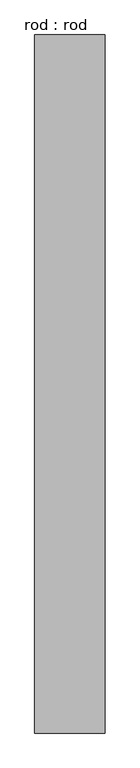
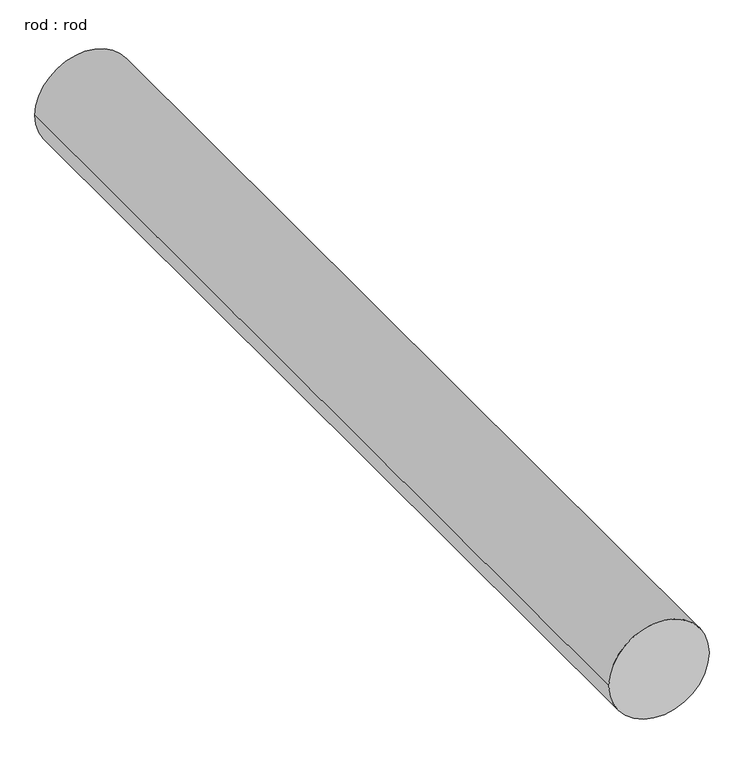
"""IFC4 building model written with IfcOpenShell, lengths in millimetres: proxy geometry, rod : rod."""

from ifc_helpers import new_model, si_unit, point, frame, frame_2d, origin, place, context, project, spatial, circle_curve, trimmed, segment, composite_curve, outline, extrude, source, transform, mapped, element, save


def rod_rod_0e9545da(model_context):
    return source(origin(), model_context, "Body", "SweptSolid", [
        extrude(outline(composite_curve([segment(trimmed(circle_curve(frame_2d((0.0108462, 0.0)), 200.0), [point((0.0108462, 200.0))], [point((0.0108462, -200.0))], False, "CARTESIAN"), True, "CONTINUOUS"), segment(trimmed(circle_curve(frame_2d((0.0108462, 0.0)), 200.0), [point((0.0108462, -200.0))], [point((0.0108462, 200.0))], False, "CARTESIAN"), True, "CONTINUOUS")], self_intersect=False)), frame((0.0, 2107.8970734, 0.0), z_axis=(0.0, 1.0, 0.0), x_axis=(0.0, 0.0, 1.0)), (0.0, 0.0, 1.0), 3969.6630839),
    ])


if __name__ == "__main__":
    model = new_model("IFC4")
    model_context = context("Model", 3, world=origin())
    ifc_project = project(units=[si_unit("LENGTHUNIT", "METRE", prefix="MILLI")], contexts=[model_context])
    site = spatial("IfcSite", under=ifc_project)
    building = spatial("IfcBuilding", under=site)
    placement = place(None, origin())
    rod_rod_shape = rod_rod_0e9545da(model_context)
    element("IfcBuildingElementProxy", 1, Name="rod : rod", ObjectType="rod : rod", at=placement, inside=building, context=model_context, shape_type="MappedRepresentation", body=[
        mapped(rod_rod_shape, transform((0.0, 0.0, 0.0), x_axis=(1.0, 0.0, 0.0), y_axis=(0.0, 1.0, 0.0), z_axis=(0.0, 0.0, 1.0))),
    ])
    save(model, "model.ifc")

# Revit data of these elements
# Type "rod : rod"
#   Default Elevation = 0
